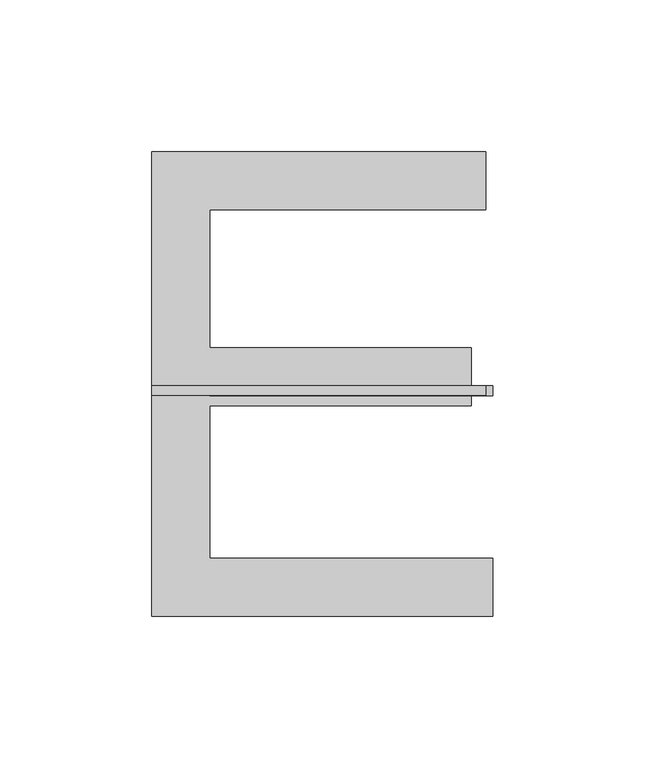
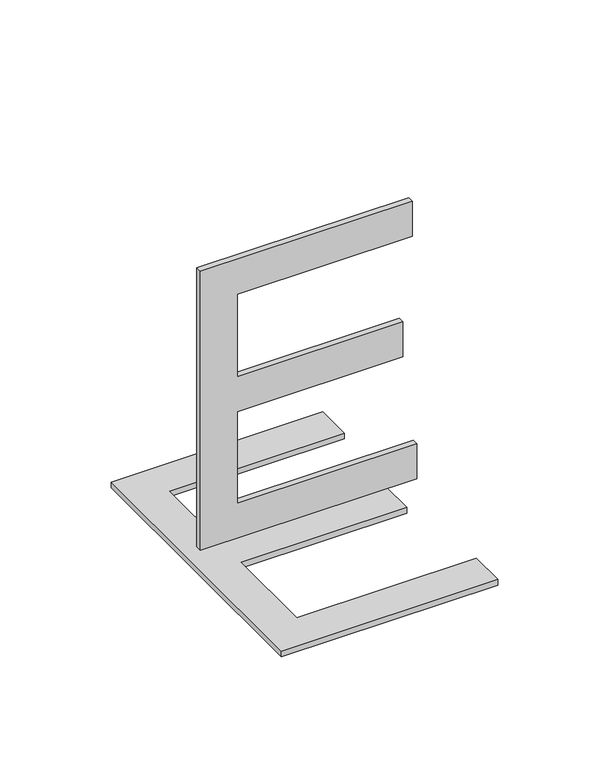
"""IFC4 building model written with IfcOpenShell, lengths in millimetres: proxy geometry, Grid Number1_FedEx : Grid Number1_FedEx."""

import ifcopenshell
import ifcopenshell.guid

model = None  # the IFC model being written
_history = None  # IfcOwnerHistory: only IFC2X3 demands one
_inside = {}  # id of a spatial element -> (the spatial element, [elements in it])
_under = {}  # id of a project, library or spatial element -> (it, [spatial elements below it])
_declared = {}  # id of a project -> (the project, [libraries it declares])
_typed = {}  # id of a type object -> (the type object, [elements of that type])
_made_of = {}  # id of a material, layer set ... -> (it, [elements and type objects made of it])


def new_model(schema):
    """Start an empty IFC model of exactly this schema.

    Asked for "IFC4X3", IfcOpenShell would pick the latest addendum, in which some entities
    have other attributes; the version numbers below select the first issue.
    IFC2X3 requires an IfcOwnerHistory on every rooted entity: one is made here for all.
    """
    global model, _history
    if schema == "IFC4X3":
        model = ifcopenshell.file(schema_version=(4, 3, 0, 0))
    else:
        model = ifcopenshell.file(schema=schema)
    _inside.clear()
    _under.clear()
    _declared.clear()
    _typed.clear()
    _made_of.clear()
    _history = None
    if model.schema == "IFC2X3":
        org = make("IfcOrganization", Name="unknown")
        user = make(
            "IfcPersonAndOrganization",
            ThePerson=make("IfcPerson", FamilyName="unknown"),
            TheOrganization=org,
        )
        app = make(
            "IfcApplication",
            ApplicationDeveloper=org,
            Version="unknown",
            ApplicationFullName="unknown",
            ApplicationIdentifier="unknown",
        )
        _history = make(
            "IfcOwnerHistory",
            OwningUser=user,
            OwningApplication=app,
            ChangeAction="ADDED",
            CreationDate=0,
        )
    return model


def make(cls, **values):
    """One entity of the class cls with the attributes given. An attribute that is None is left unset."""
    return model.create_entity(
        cls, **{name: value for name, value in values.items() if value is not None}
    )


def rooted(cls, **values):
    """An entity with a GlobalId (a new one), such as an element, a storey or a relation."""
    return make(cls, GlobalId=ifcopenshell.guid.new(), OwnerHistory=_history, **values)


def si_unit(unit_type, name, prefix=None):
    """IfcSIUnit, for example si_unit("LENGTHUNIT", "METRE", prefix="MILLI")."""
    return make("IfcSIUnit", UnitType=unit_type, Prefix=prefix, Name=name)


def assignment(units):
    """IfcUnitAssignment: the units of a project."""
    return None if units is None else make("IfcUnitAssignment", Units=units)


def point(xyz):
    """IfcCartesianPoint."""
    return None if xyz is None else make("IfcCartesianPoint", Coordinates=xyz)


def direction(xyz):
    """IfcDirection."""
    return None if xyz is None else make("IfcDirection", DirectionRatios=xyz)


def frame(location, z_axis=None, x_axis=None):
    """IfcAxis2Placement3D, a coordinate frame: its origin and axes. An axis left out is left unset."""
    return make(
        "IfcAxis2Placement3D",
        Location=point(location),
        Axis=direction(z_axis),
        RefDirection=direction(x_axis),
    )


def origin():
    """The frame at (0, 0, 0) with its axes left unset."""
    return frame((0.0, 0.0, 0.0))


def origin_with_axes():
    """The frame at (0, 0, 0) with the z axis (0, 0, 1) and the x axis (1, 0, 0) written out."""
    return frame((0.0, 0.0, 0.0), z_axis=(0.0, 0.0, 1.0), x_axis=(1.0, 0.0, 0.0))


def place(relative_to, where):
    """IfcLocalPlacement: puts the frame where relative to a parent placement (None: the world)."""
    return make(
        "IfcLocalPlacement", PlacementRelTo=relative_to, RelativePlacement=where
    )


def context(
    kind, dimensions, precision=None, world=None, true_north=None, identifier=None
):
    """IfcGeometricRepresentationContext, for example the 3D "Model" context."""
    return make(
        "IfcGeometricRepresentationContext",
        ContextIdentifier=identifier,
        ContextType=kind,
        CoordinateSpaceDimension=dimensions,
        Precision=precision,
        WorldCoordinateSystem=world,
        TrueNorth=true_north,
    )


def project(units=None, contexts=None):
    """IfcProject with its units and contexts."""
    return rooted(
        "IfcProject",
        Name="project",
        RepresentationContexts=contexts,
        UnitsInContext=assignment(units),
    )


def spatial(cls, under=None, at=None, **own):
    """A site, building, storey or space (cls), placed at a placement, below another one or the project."""
    s = rooted(cls, ObjectPlacement=at, **own)
    if under is not None:
        _under.setdefault(under.id(), (under, []))[1].append(s)
    return s


def polyline(points):
    """IfcPolyline through the points."""
    return make("IfcPolyline", Points=[point(p) for p in points])


def outline(outer, holes=None, kind="AREA"):
    """IfcArbitraryClosedProfileDef: a profile drawn as a closed curve; with holes, ...WithVoids."""
    if holes is None:
        return make("IfcArbitraryClosedProfileDef", ProfileType=kind, OuterCurve=outer)
    return make(
        "IfcArbitraryProfileDefWithVoids",
        ProfileType=kind,
        OuterCurve=outer,
        InnerCurves=holes,
    )


def extrude(swept, where, along, depth):
    """IfcExtrudedAreaSolid: the profile swept, set in the frame where, extruded along a direction by depth."""
    return make(
        "IfcExtrudedAreaSolid",
        SweptArea=swept,
        Position=where,
        ExtrudedDirection=direction(along),
        Depth=depth,
    )


def shape(context_of_items, identifier, shape_type, items):
    """IfcShapeRepresentation: the items that make up one representation, for example the "Body"."""
    return make(
        "IfcShapeRepresentation",
        ContextOfItems=context_of_items,
        RepresentationIdentifier=identifier,
        RepresentationType=shape_type,
        Items=items,
    )


def source(mapping_origin, context_of_items, identifier, shape_type, items):
    """IfcRepresentationMap: a shape defined once, which mapped items show again and again."""
    return make(
        "IfcRepresentationMap",
        MappingOrigin=mapping_origin,
        MappedRepresentation=shape(context_of_items, identifier, shape_type, items),
    )


def transform(
    local_origin,
    x_axis=None,
    y_axis=None,
    z_axis=None,
    scale=None,
    scale2=None,
    scale3=None,
    uniform=True,
):
    """IfcCartesianTransformationOperator3D, or its non-uniform kind. x_axis, y_axis, z_axis: its Axis1, 2, 3."""
    if uniform:
        return make(
            "IfcCartesianTransformationOperator3D",
            Axis1=direction(x_axis),
            Axis2=direction(y_axis),
            LocalOrigin=point(local_origin),
            Scale=scale,
            Axis3=direction(z_axis),
        )
    return make(
        "IfcCartesianTransformationOperator3DnonUniform",
        Axis1=direction(x_axis),
        Axis2=direction(y_axis),
        LocalOrigin=point(local_origin),
        Scale=scale,
        Axis3=direction(z_axis),
        Scale2=scale2,
        Scale3=scale3,
    )


def mapped(mapping_source, mapping_target):
    """IfcMappedItem: shows the shape of a source again, moved by a transform."""
    return make(
        "IfcMappedItem", MappingSource=mapping_source, MappingTarget=mapping_target
    )


def made_of(thing, what):
    """Note that an element or type object is made of a material, layer set ...; save() writes the relation."""
    if what is not None:
        _made_of.setdefault(what.id(), (what, []))[1].append(thing)
    return thing


def element(
    cls,
    number,
    at=None,
    inside=None,
    cuts=None,
    type_object=None,
    material=None,
    context=None,
    identifier="Body",
    shape_type=None,
    held_by="IfcProductDefinitionShape",
    body=None,
    shapes=None,
    **own,
):
    """One element of the class cls, such as IfcWall. Its Tag is "e" and its number.

    at: its placement. inside: the storey or other place that contains it. cuts: it is an
    opening in that element (IfcRelVoidsElement). A single representation is given by context,
    identifier, shape_type and body (its items); several are given by shapes. held_by: the class
    of the entity that holds the representations. save() writes the other relations.
    """
    e = rooted(cls, Tag="e%d" % number, ObjectPlacement=at, **own)
    if body is not None:
        shapes = [shape(context, identifier, shape_type, body)]
    if shapes is not None:
        e.Representation = make(held_by, Representations=shapes)
    if inside is not None:
        _inside.setdefault(inside.id(), (inside, []))[1].append(e)
    if cuts is not None:
        rooted(
            "IfcRelVoidsElement", RelatingBuildingElement=cuts, RelatedOpeningElement=e
        )
    if type_object is not None:
        _typed.setdefault(type_object.id(), (type_object, []))[1].append(e)
    return made_of(e, material)


def aggregate(whole, parts):
    """IfcRelAggregates: a whole, such as a stair, and the parts it consists of."""
    return rooted("IfcRelAggregates", RelatingObject=whole, RelatedObjects=parts)


def save(model, path):
    """Write the relations noted so far, then the file.

    IfcRelAggregates (storeys below a building ...), IfcRelContainedInSpatialStructure (elements
    in a storey), IfcRelDefinesByType, IfcRelAssociatesMaterial and IfcRelDeclares: one each for
    every whole, place, type object, material and project.
    """
    for whole, parts in _under.values():
        aggregate(whole, parts)
    for where, things in _inside.values():
        rooted(
            "IfcRelContainedInSpatialStructure",
            RelatedElements=things,
            RelatingStructure=where,
        )
    for kind, things in _typed.values():
        rooted("IfcRelDefinesByType", RelatedObjects=things, RelatingType=kind)
    for what, things in _made_of.values():
        rooted("IfcRelAssociatesMaterial", RelatedObjects=things, RelatingMaterial=what)
    for by, libraries in _declared.values():
        rooted("IfcRelDeclares", RelatingContext=by, RelatedDefinitions=libraries)
    model.write(path)


def entourage_efcd05c0(model_context):
    return source(origin(), model_context, "Body", "SweptSolid", [
        extrude(outline(polyline([(-161.8965342, 146.5840649), (-161.8965342, 299.6794816), (-51.8592034, 299.6794816), (-51.8592034, 280.5425545), (-142.7596071, 280.5425545), (-142.7596071, 235.0923527), (-56.6434352, 235.0923527), (-56.6434352, 215.9554256), (-142.7596071, 215.9554256), (-142.7596071, 165.720992), (-49.4670875, 165.720992), (-49.4670875, 146.5840649), (-161.8965342, 146.5840649)])), origin_with_axes(), (0.0, 0.0, 1.0), 3.175),
        extrude(outline(polyline([(14.4798932, -161.8965342), (14.4798932, -49.4670875), (33.6168203, -49.4670875), (33.6168203, -142.7596071), (83.8512539, -142.7596071), (83.8512539, -56.6434352), (102.988181, -56.6434352), (102.988181, -142.7596071), (148.4383828, -142.7596071), (148.4383828, -51.8592034), (167.5753099, -51.8592034), (167.5753099, -161.8965342), (14.4798932, -161.8965342)])), frame((0.0, 219.3456765, 0.0), z_axis=(0.0, 1.0, 0.0), x_axis=(0.0, 0.0, 1.0)), (0.0, 0.0, 1.0), 3.175),
    ])


if __name__ == "__main__":
    model = new_model("IFC4")
    model_context = context("Model", 3, world=origin())
    ifc_project = project(units=[si_unit("LENGTHUNIT", "METRE", prefix="MILLI")], contexts=[model_context])
    site = spatial("IfcSite", under=ifc_project)
    building = spatial("IfcBuilding", under=site)
    placement = place(None, origin())
    entourage_shape = entourage_efcd05c0(model_context)
    element("IfcBuildingElementProxy", 1, Name="Grid Number1_FedEx : Grid Number1_FedEx", ObjectType="Grid Number1_FedEx : Grid Number1_FedEx", at=placement, inside=building, context=model_context, shape_type="MappedRepresentation", body=[
        mapped(entourage_shape, transform((0.0, 0.0, 0.0), x_axis=(1.0, 0.0, 0.0), y_axis=(0.0, 1.0, 0.0), z_axis=(0.0, 0.0, 1.0))),
    ])
    save(model, "model.ifc")

# Revit data of these elements
# Type "Grid Number1_FedEx : Grid Number1_FedEx"
#   Grid [instance default] = "S.8"
#   Label Width [instance default] = 1' - 0"
#   Half Box Width2 [instance default] = 0' - 6.13846"
#   Half Box Width [instance default] = 0' - 6"
#   Robust [instance default] = yes
#   Height = 0
#   Assembly Code = ""
# Element 1 (IfcBuildingElementProxy, "Grid Number1_FedEx : Grid Number1_FedEx")
#   Grid = "E"
#   Robust = no
#   Materials on its faces: "Letter"
# Materials
#   "Letter": class "Unassigned", colour RGB 178 187 30, transparency 0, Comments = "Rendering appearance not upgraded "
